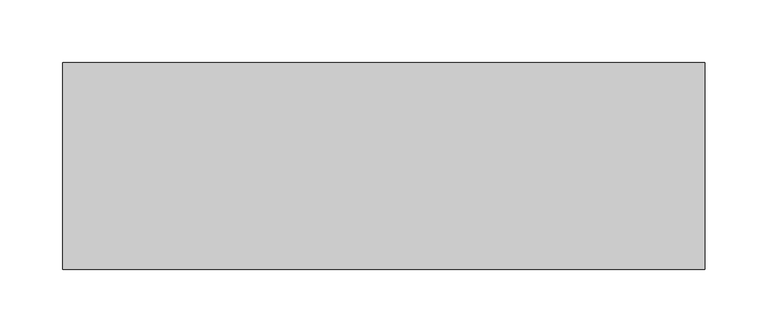
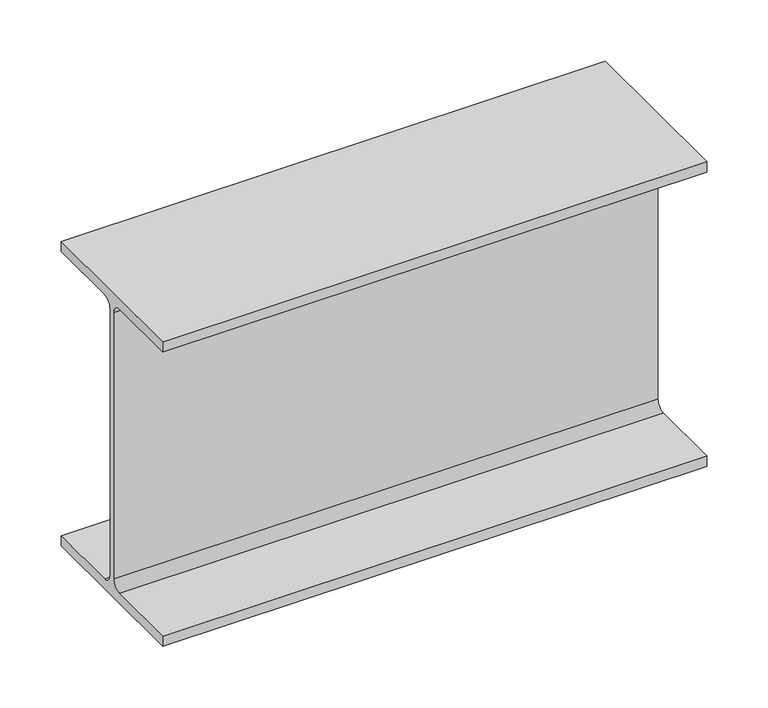
"""IFC4 building model written with IfcOpenShell, lengths in millimetres: beam geometry, Steel Beam_H-KSD3502 : H_SB_ASB_H-300x150x6.5x9."""

from ifc_helpers import new_model, si_unit, point, frame, frame_2d, origin, place, context, project, spatial, polyline, circle_curve, trimmed, segment, composite_curve, outline, extrude, source, transform, mapped, element, save


def beam_abe9414c(model_context):
    return source(origin(), model_context, "Body", "SweptSolid", [
        extrude(outline(composite_curve([segment(polyline([(82.5, -141.5), (82.5, -151.7), (-82.5, -151.7), (-82.5, -141.5), (-11.9, -141.5)]), True, "CONTINUOUS"), segment(trimmed(circle_curve(frame_2d((-11.9, -132.6)), 8.9), [point((-11.9, -141.5))], [point((-3.0, -132.6))], True, "CARTESIAN"), True, "CONTINUOUS"), segment(polyline([(-3.0, -132.6), (-3.0, 132.6)]), True, "CONTINUOUS"), segment(trimmed(circle_curve(frame_2d((-11.9, 132.6)), 8.9), [point((-3.0, 132.6))], [point((-11.9, 141.5))], True, "CARTESIAN"), True, "CONTINUOUS"), segment(polyline([(-11.9, 141.5), (-82.5, 141.5), (-82.5, 151.7), (82.5, 151.7), (82.5, 141.5), (11.9, 141.5)]), True, "CONTINUOUS"), segment(trimmed(circle_curve(frame_2d((11.9, 132.6)), 8.9), [point((11.9, 141.5))], [point((3.0, 132.6))], True, "CARTESIAN"), True, "CONTINUOUS"), segment(polyline([(3.0, 132.6), (3.0, -132.6)]), True, "CONTINUOUS"), segment(trimmed(circle_curve(frame_2d((11.9, -132.6)), 8.9), [point((3.0, -132.6))], [point((11.9, -141.5))], True, "CARTESIAN"), True, "CONTINUOUS"), segment(polyline([(11.9, -141.5), (82.5, -141.5)]), True, "CONTINUOUS")], self_intersect=False)), frame((-300.0, 0.0, 0.0), z_axis=(1.0, 0.0, 0.0), x_axis=(0.0, 1.0, 0.0)), (0.0, 0.0, 1.0), 512.3),
    ])


if __name__ == "__main__":
    model = new_model("IFC4")
    model_context = context("Model", 3, world=origin())
    ifc_project = project(units=[si_unit("LENGTHUNIT", "METRE", prefix="MILLI")], contexts=[model_context])
    site = spatial("IfcSite", under=ifc_project)
    building = spatial("IfcBuilding", under=site)
    placement = place(None, origin())
    beam_shape = beam_abe9414c(model_context)
    element("IfcBeam", 1, ObjectType="Steel Beam_H-KSD3502 : H_SB_ASB_H-300x150x6.5x9", at=placement, inside=building, context=model_context, shape_type="MappedRepresentation", body=[
        mapped(beam_shape, transform((0.0, 0.0, 0.0), x_axis=(1.0, 0.0, 0.0), y_axis=(0.0, 1.0, 0.0), z_axis=(0.0, 0.0, 1.0))),
    ])
    save(model, "model.ifc")

# Revit data of these elements
# Type "Steel Beam_H-KSD3502 : H_SB_ASB_H-300x150x6.5x9"
#   Width = 15.0 cm
#   Web Thickness = 0.65 cm
#   Web Fillet = 1.3 cm
#   Warping Constant = 107174.0 cm⁶
#   Torsional Moment of Inertia = 9.9539 cm⁴
#   Torsional Modulus = 1.0 cm³
#   Section Area = 46.78 cm²
#   Plastic Modulus weak axis = 105.0 cm³
#   Plastic Modulus strong axis = 542.0 cm³
#   Perimeter = 1.17 m²/m
#   Nominal Weight = 36.70 kgf/m
#   Moment of Inertia weak axis = 508.00 cm⁴
#   Moment of Inertia strong axis = 7210.00 cm⁴
#   Height = 30.0 cm
#   Flange Thickness = 0.9 cm
#   Elastic Modulus weak axis = 67.7 cm³
#   Elastic Modulus strong axis = 481.0 cm³
#   Centroid Vertical = 15.0 cm
#   Centroid Horizontal = 7.5 cm
#   Length [instance default] = 1.5240 m
#   Structural Material [instance default] = Steel, 45-345
#   Assembly Code = ""
# Element 1 (IfcBeam, "Steel Beam_H-KSD3502 : H_SB_ASB_H-300x150x6.5x9")
#   Structural Material = none
# Materials
#   "Steel, 45-345": class "Metal", colour RGB 189 187 185, transparency 0, Description = "Steel 345 MPa", Cost = 0
